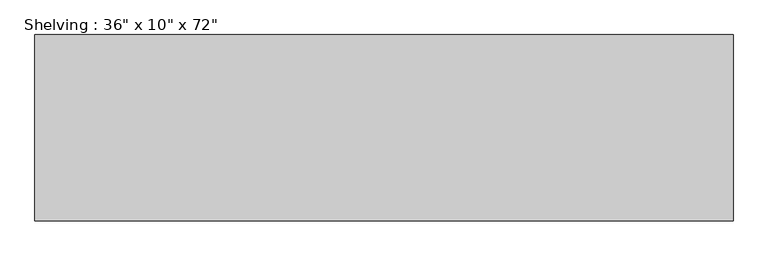
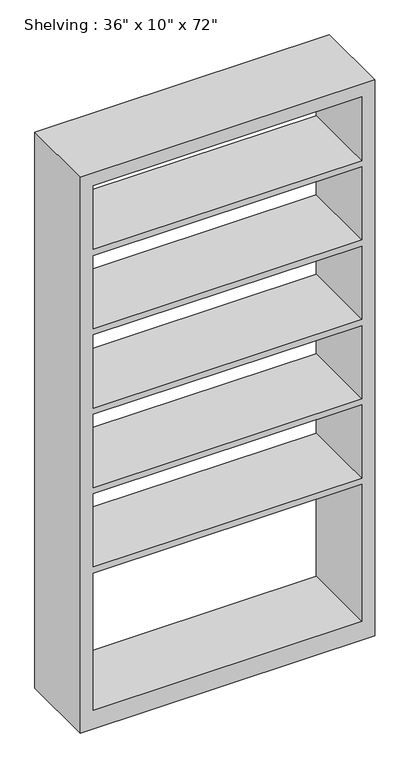
"""IFC4 building model written with IfcOpenShell, lengths in millimetres: furniture geometry."""

from ifc_helpers import new_model, si_unit, frame, origin, place, context, project, spatial, polyline, outline, extrude, source, transform, mapped, element, save


def furniture_cabf2c48(model_context):
    return source(origin(), model_context, "Body", "SweptSolid", [
        extrude(outline(polyline([(0.0, 571.5), (2279.65, 571.5), (2279.65, -571.5), (0.0, -571.5), (0.0, 571.5)]), holes=[polyline([(2228.85, 520.7), (1966.6857143, 520.7), (1966.6857143, -520.7), (2228.85, -520.7), (2228.85, 520.7)]), polyline([(76.2, 520.7), (76.2, -520.7), (638.6285714, -520.7), (638.6285714, 520.7), (76.2, 520.7)]), polyline([(1315.3571429, -520.7), (1615.6214286, -520.7), (1615.6214286, 520.7), (1315.3571429, 520.7), (1315.3571429, -520.7)]), polyline([(1941.2857143, 520.7), (1641.0214286, 520.7), (1641.0214286, -520.7), (1941.2857143, -520.7), (1941.2857143, 520.7)]), polyline([(1289.9571429, 520.7), (989.6928571, 520.7), (989.6928571, -520.7), (1289.9571429, -520.7), (1289.9571429, 520.7)]), polyline([(964.2928571, 520.7), (664.0285714, 520.7), (664.0285714, -520.7), (964.2928571, -520.7), (964.2928571, 520.7)])]), frame((0.0, -457.2, 0.0), z_axis=(0.0, 1.0, 0.0), x_axis=(0.0, 0.0, 1.0)), (0.0, 0.0, 1.0), 304.8),
    ])


if __name__ == "__main__":
    model = new_model("IFC4")
    model_context = context("Model", 3, world=origin())
    ifc_project = project(units=[si_unit("LENGTHUNIT", "METRE", prefix="MILLI")], contexts=[model_context])
    site = spatial("IfcSite", under=ifc_project)
    building = spatial("IfcBuilding", under=site)
    placement = place(None, origin())
    furniture_shape = furniture_cabf2c48(model_context)
    element("IfcFurniture", 1, ObjectType="Shelving : 36\" x 10\" x 72\"", at=placement, inside=building, context=model_context, shape_type="MappedRepresentation", body=[
        mapped(furniture_shape, transform((0.0, 0.0, 0.0), x_axis=(1.0, 0.0, 0.0), y_axis=(0.0, 1.0, 0.0), z_axis=(0.0, 0.0, 1.0))),
    ])
    save(model, "model.ifc")

# Revit data of these elements
# Type "Shelving : 36\" x 10\" x 72\""
#   Assembly Code = "E2020200"
#   Depth = 1' - 0"
#   Height = 7' - 5 3/4"
#   Width = 3' - 9"
#   Shelving Unit Material = Wood - Birch
# Element 1 (IfcFurniture, "Shelving : 36\" x 10\" x 72\"")
#   Materials on its faces: "Wood - Birch"
# Materials
#   "Wood - Birch": class "Wood", colour RGB 224 178 126, transparency 0
